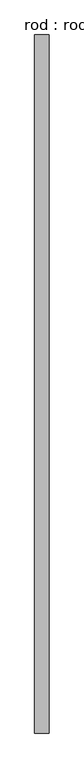
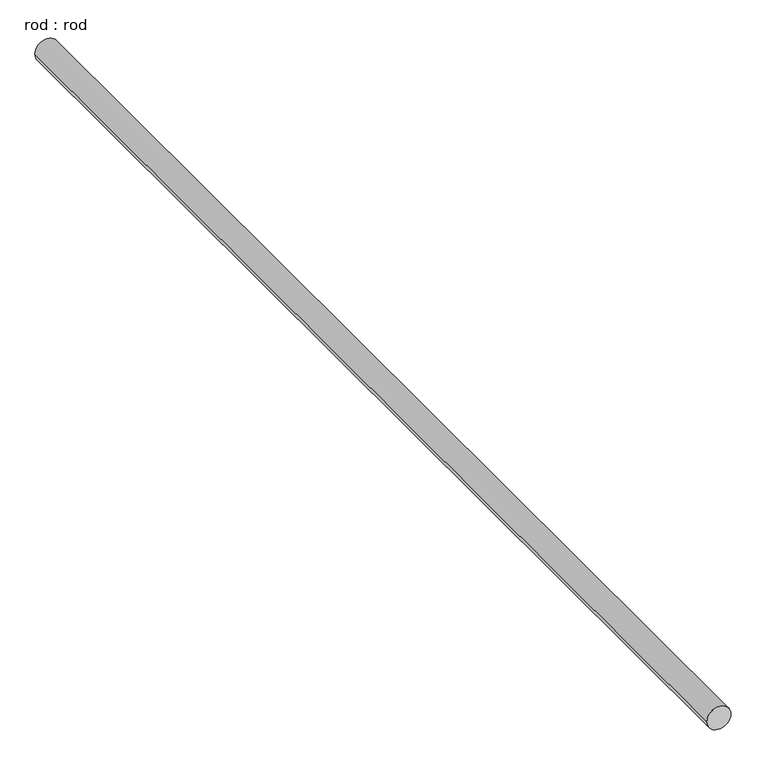
"""IFC4 building model written with IfcOpenShell, lengths in millimetres: proxy geometry, rod : rod."""

from ifc_helpers import new_model, si_unit, point, frame, frame_2d, origin, place, context, project, spatial, circle_curve, trimmed, segment, composite_curve, outline, extrude, source, transform, mapped, element, save


def rod_rod_83c0bad8(model_context):
    return source(origin(), model_context, "Body", "SweptSolid", [
        extrude(outline(composite_curve([segment(trimmed(circle_curve(frame_2d((0.0108462, 0.0)), 200.0), [point((0.0108462, 200.0))], [point((0.0108462, -200.0))], False, "CARTESIAN"), True, "CONTINUOUS"), segment(trimmed(circle_curve(frame_2d((0.0108462, 0.0)), 200.0), [point((0.0108462, -200.0))], [point((0.0108462, 200.0))], False, "CARTESIAN"), True, "CONTINUOUS")], self_intersect=False)), frame((0.0, -5638.8337592, 0.0), z_axis=(0.0, 1.0, 0.0), x_axis=(0.0, 0.0, 1.0)), (0.0, 0.0, 1.0), 19463.1247491),
    ])


if __name__ == "__main__":
    model = new_model("IFC4")
    model_context = context("Model", 3, world=origin())
    ifc_project = project(units=[si_unit("LENGTHUNIT", "METRE", prefix="MILLI")], contexts=[model_context])
    site = spatial("IfcSite", under=ifc_project)
    building = spatial("IfcBuilding", under=site)
    placement = place(None, origin())
    rod_rod_shape = rod_rod_83c0bad8(model_context)
    element("IfcBuildingElementProxy", 1, Name="rod : rod", ObjectType="rod : rod", at=placement, inside=building, context=model_context, shape_type="MappedRepresentation", body=[
        mapped(rod_rod_shape, transform((0.0, 0.0, 0.0), x_axis=(1.0, 0.0, 0.0), y_axis=(0.0, 1.0, 0.0), z_axis=(0.0, 0.0, 1.0))),
    ])
    save(model, "model.ifc")

# Revit data of these elements
# Type "rod : rod"
#   Default Elevation = 0
